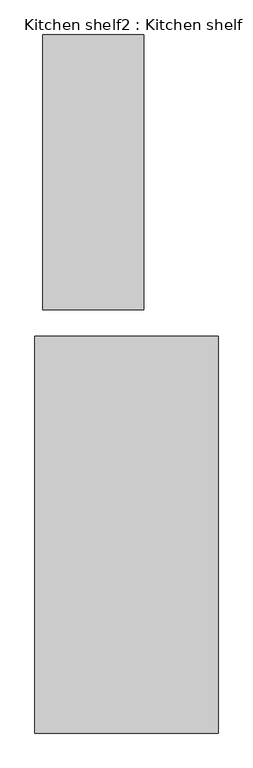
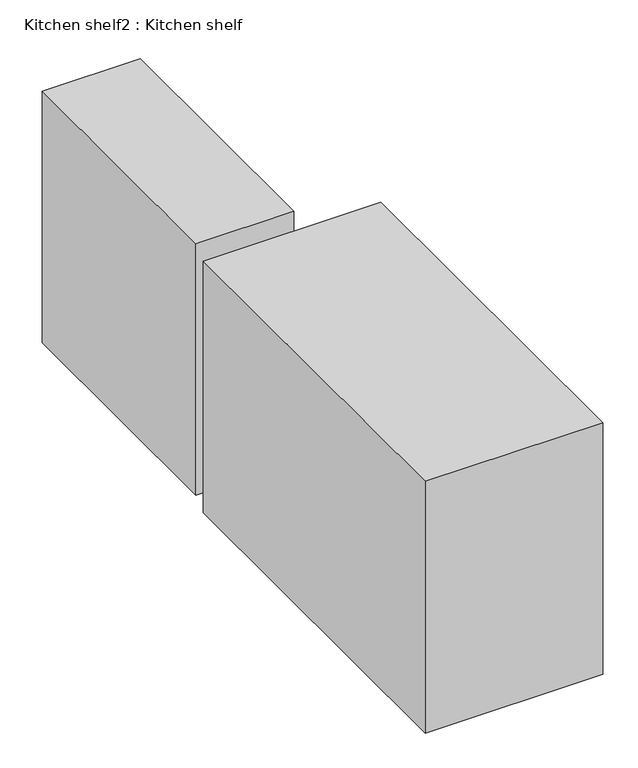
"""IFC4 building model written with IfcOpenShell, lengths in millimetres: furniture geometry, Kitchen shelf2 : Kitchen shelf."""

from ifc_helpers import new_model, si_unit, origin, origin_with_axes, place, context, project, spatial, polyline, outline, extrude, source, transform, mapped, element, save


def kitchen_shelf2_kitchen_shelf_433be29b(model_context):
    return source(origin(), model_context, "Body", "SweptSolid", [
        extrude(outline(polyline([(23330.3768331, 864.8615366), (23330.3768331, -49.5384634), (22994.1370052, -49.5384634), (22994.1370052, 864.8615366), (23330.3768331, 864.8615366)])), origin_with_axes(), (0.0, 0.0, 1.0), 914.4),
        extrude(outline(polyline([(22968.7370052, -138.4384634), (23578.3370052, -138.4384634), (23578.3370052, -1459.2384634), (22968.7370052, -1459.2384634), (22968.7370052, -138.4384634)])), origin_with_axes(), (0.0, 0.0, 1.0), 914.4),
    ])


if __name__ == "__main__":
    model = new_model("IFC4")
    model_context = context("Model", 3, world=origin())
    ifc_project = project(units=[si_unit("LENGTHUNIT", "METRE", prefix="MILLI")], contexts=[model_context])
    site = spatial("IfcSite", under=ifc_project)
    building = spatial("IfcBuilding", under=site)
    placement = place(None, origin())
    kitchen_shelf2_kitchen_shelf_shape = kitchen_shelf2_kitchen_shelf_433be29b(model_context)
    element("IfcFurniture", 1, ObjectType="Kitchen shelf2 : Kitchen shelf", at=placement, inside=building, context=model_context, shape_type="MappedRepresentation", body=[
        mapped(kitchen_shelf2_kitchen_shelf_shape, transform((0.0, 0.0, 0.0), x_axis=(1.0, 0.0, 0.0), y_axis=(0.0, 1.0, 0.0), z_axis=(0.0, 0.0, 1.0))),
    ])
    save(model, "model.ifc")
